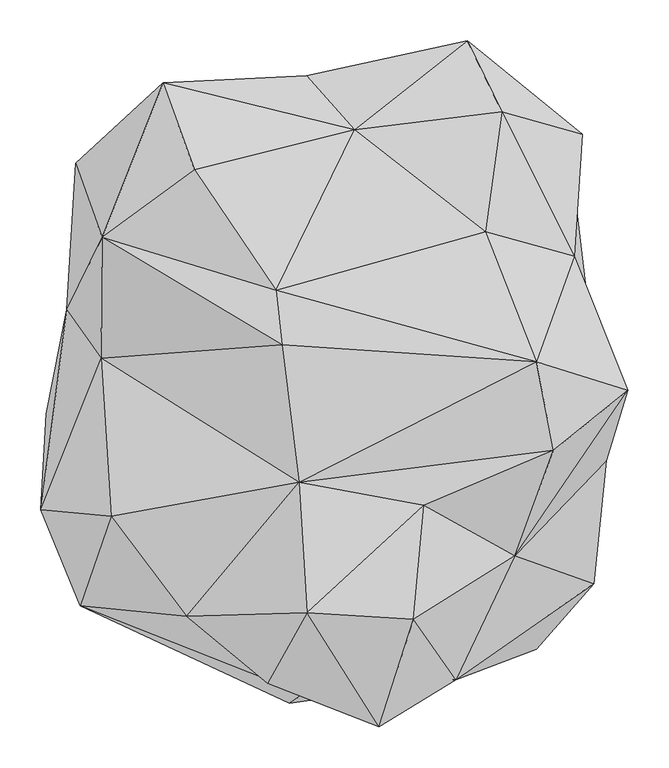
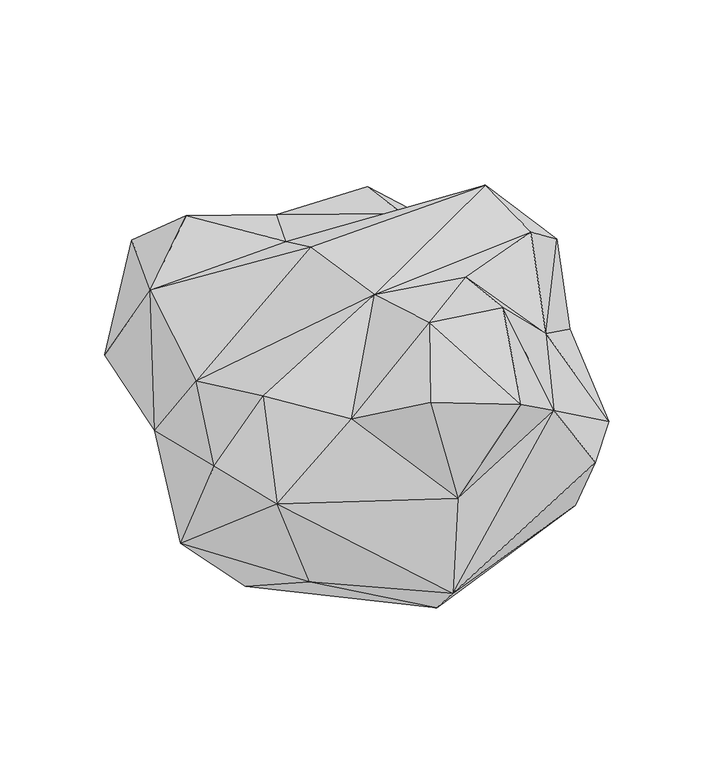
"""IFC4 building model written with IfcOpenShell, lengths in millimetres: geographic element geometry, Enscape AssetDefinition - Asparagaceae 001 Agave : Enscape AssetDefinition - Asparagaceae 001 Agave."""

import ifcopenshell
import ifcopenshell.guid

model = None  # the IFC model being written
_history = None  # IfcOwnerHistory: only IFC2X3 demands one
_inside = {}  # id of a spatial element -> (the spatial element, [elements in it])
_under = {}  # id of a project, library or spatial element -> (it, [spatial elements below it])
_declared = {}  # id of a project -> (the project, [libraries it declares])
_typed = {}  # id of a type object -> (the type object, [elements of that type])
_made_of = {}  # id of a material, layer set ... -> (it, [elements and type objects made of it])


def new_model(schema):
    """Start an empty IFC model of exactly this schema.

    Asked for "IFC4X3", IfcOpenShell would pick the latest addendum, in which some entities
    have other attributes; the version numbers below select the first issue.
    IFC2X3 requires an IfcOwnerHistory on every rooted entity: one is made here for all.
    """
    global model, _history
    if schema == "IFC4X3":
        model = ifcopenshell.file(schema_version=(4, 3, 0, 0))
    else:
        model = ifcopenshell.file(schema=schema)
    _inside.clear()
    _under.clear()
    _declared.clear()
    _typed.clear()
    _made_of.clear()
    _history = None
    if model.schema == "IFC2X3":
        org = make("IfcOrganization", Name="unknown")
        user = make(
            "IfcPersonAndOrganization",
            ThePerson=make("IfcPerson", FamilyName="unknown"),
            TheOrganization=org,
        )
        app = make(
            "IfcApplication",
            ApplicationDeveloper=org,
            Version="unknown",
            ApplicationFullName="unknown",
            ApplicationIdentifier="unknown",
        )
        _history = make(
            "IfcOwnerHistory",
            OwningUser=user,
            OwningApplication=app,
            ChangeAction="ADDED",
            CreationDate=0,
        )
    return model


def make(cls, **values):
    """One entity of the class cls with the attributes given. An attribute that is None is left unset."""
    return model.create_entity(
        cls, **{name: value for name, value in values.items() if value is not None}
    )


def rooted(cls, **values):
    """An entity with a GlobalId (a new one), such as an element, a storey or a relation."""
    return make(cls, GlobalId=ifcopenshell.guid.new(), OwnerHistory=_history, **values)


def si_unit(unit_type, name, prefix=None):
    """IfcSIUnit, for example si_unit("LENGTHUNIT", "METRE", prefix="MILLI")."""
    return make("IfcSIUnit", UnitType=unit_type, Prefix=prefix, Name=name)


def assignment(units):
    """IfcUnitAssignment: the units of a project."""
    return None if units is None else make("IfcUnitAssignment", Units=units)


def point(xyz):
    """IfcCartesianPoint."""
    return None if xyz is None else make("IfcCartesianPoint", Coordinates=xyz)


def direction(xyz):
    """IfcDirection."""
    return None if xyz is None else make("IfcDirection", DirectionRatios=xyz)


def frame(location, z_axis=None, x_axis=None):
    """IfcAxis2Placement3D, a coordinate frame: its origin and axes. An axis left out is left unset."""
    return make(
        "IfcAxis2Placement3D",
        Location=point(location),
        Axis=direction(z_axis),
        RefDirection=direction(x_axis),
    )


def origin():
    """The frame at (0, 0, 0) with its axes left unset."""
    return frame((0.0, 0.0, 0.0))


def place(relative_to, where):
    """IfcLocalPlacement: puts the frame where relative to a parent placement (None: the world)."""
    return make(
        "IfcLocalPlacement", PlacementRelTo=relative_to, RelativePlacement=where
    )


def context(
    kind, dimensions, precision=None, world=None, true_north=None, identifier=None
):
    """IfcGeometricRepresentationContext, for example the 3D "Model" context."""
    return make(
        "IfcGeometricRepresentationContext",
        ContextIdentifier=identifier,
        ContextType=kind,
        CoordinateSpaceDimension=dimensions,
        Precision=precision,
        WorldCoordinateSystem=world,
        TrueNorth=true_north,
    )


def project(units=None, contexts=None):
    """IfcProject with its units and contexts."""
    return rooted(
        "IfcProject",
        Name="project",
        RepresentationContexts=contexts,
        UnitsInContext=assignment(units),
    )


def spatial(cls, under=None, at=None, **own):
    """A site, building, storey or space (cls), placed at a placement, below another one or the project."""
    s = rooted(cls, ObjectPlacement=at, **own)
    if under is not None:
        _under.setdefault(under.id(), (under, []))[1].append(s)
    return s


def faces_of(points, faces, orient=None, outer=None):
    """IfcFace entities. A face is a list of loops; a loop is a list of indices into points, from 0.

    orient and outer hold one flag for each loop. By default every Orientation is true, the
    first loop of a face is its IfcFaceOuterBound and the others are IfcFaceBound.
    """
    made = []
    for i, loops in enumerate(faces):
        bounds = []
        for j, loop in enumerate(loops):
            is_outer = j == 0 if outer is None else outer[i][j]
            bounds.append(
                make(
                    "IfcFaceOuterBound" if is_outer else "IfcFaceBound",
                    Bound=make("IfcPolyLoop", Polygon=[points[k] for k in loop]),
                    Orientation=True if orient is None else orient[i][j],
                )
            )
        made.append(make("IfcFace", Bounds=bounds))
    return made


def faceted_brep(points, faces, orient=None, outer=None, voids=None):
    """IfcFacetedBrep: a solid bounded by flat faces; with voids (closed shells), ...WithVoids."""
    shared = [point(p) for p in points]
    hull = make("IfcClosedShell", CfsFaces=faces_of(shared, faces, orient, outer))
    if voids is None:
        return make("IfcFacetedBrep", Outer=hull)
    return make(
        "IfcFacetedBrepWithVoids",
        Outer=hull,
        Voids=[
            make(cls, CfsFaces=faces_of(shared, fs, o, b)) for cls, fs, o, b in voids
        ],
    )


def shape(context_of_items, identifier, shape_type, items):
    """IfcShapeRepresentation: the items that make up one representation, for example the "Body"."""
    return make(
        "IfcShapeRepresentation",
        ContextOfItems=context_of_items,
        RepresentationIdentifier=identifier,
        RepresentationType=shape_type,
        Items=items,
    )


def source(mapping_origin, context_of_items, identifier, shape_type, items):
    """IfcRepresentationMap: a shape defined once, which mapped items show again and again."""
    return make(
        "IfcRepresentationMap",
        MappingOrigin=mapping_origin,
        MappedRepresentation=shape(context_of_items, identifier, shape_type, items),
    )


def transform(
    local_origin,
    x_axis=None,
    y_axis=None,
    z_axis=None,
    scale=None,
    scale2=None,
    scale3=None,
    uniform=True,
):
    """IfcCartesianTransformationOperator3D, or its non-uniform kind. x_axis, y_axis, z_axis: its Axis1, 2, 3."""
    if uniform:
        return make(
            "IfcCartesianTransformationOperator3D",
            Axis1=direction(x_axis),
            Axis2=direction(y_axis),
            LocalOrigin=point(local_origin),
            Scale=scale,
            Axis3=direction(z_axis),
        )
    return make(
        "IfcCartesianTransformationOperator3DnonUniform",
        Axis1=direction(x_axis),
        Axis2=direction(y_axis),
        LocalOrigin=point(local_origin),
        Scale=scale,
        Axis3=direction(z_axis),
        Scale2=scale2,
        Scale3=scale3,
    )


def mapped(mapping_source, mapping_target):
    """IfcMappedItem: shows the shape of a source again, moved by a transform."""
    return make(
        "IfcMappedItem", MappingSource=mapping_source, MappingTarget=mapping_target
    )


def made_of(thing, what):
    """Note that an element or type object is made of a material, layer set ...; save() writes the relation."""
    if what is not None:
        _made_of.setdefault(what.id(), (what, []))[1].append(thing)
    return thing


def element(
    cls,
    number,
    at=None,
    inside=None,
    cuts=None,
    type_object=None,
    material=None,
    context=None,
    identifier="Body",
    shape_type=None,
    held_by="IfcProductDefinitionShape",
    body=None,
    shapes=None,
    **own,
):
    """One element of the class cls, such as IfcWall. Its Tag is "e" and its number.

    at: its placement. inside: the storey or other place that contains it. cuts: it is an
    opening in that element (IfcRelVoidsElement). A single representation is given by context,
    identifier, shape_type and body (its items); several are given by shapes. held_by: the class
    of the entity that holds the representations. save() writes the other relations.
    """
    e = rooted(cls, Tag="e%d" % number, ObjectPlacement=at, **own)
    if body is not None:
        shapes = [shape(context, identifier, shape_type, body)]
    if shapes is not None:
        e.Representation = make(held_by, Representations=shapes)
    if inside is not None:
        _inside.setdefault(inside.id(), (inside, []))[1].append(e)
    if cuts is not None:
        rooted(
            "IfcRelVoidsElement", RelatingBuildingElement=cuts, RelatedOpeningElement=e
        )
    if type_object is not None:
        _typed.setdefault(type_object.id(), (type_object, []))[1].append(e)
    return made_of(e, material)


def aggregate(whole, parts):
    """IfcRelAggregates: a whole, such as a stair, and the parts it consists of."""
    return rooted("IfcRelAggregates", RelatingObject=whole, RelatedObjects=parts)


def save(model, path):
    """Write the relations noted so far, then the file.

    IfcRelAggregates (storeys below a building ...), IfcRelContainedInSpatialStructure (elements
    in a storey), IfcRelDefinesByType, IfcRelAssociatesMaterial and IfcRelDeclares: one each for
    every whole, place, type object, material and project.
    """
    for whole, parts in _under.values():
        aggregate(whole, parts)
    for where, things in _inside.values():
        rooted(
            "IfcRelContainedInSpatialStructure",
            RelatedElements=things,
            RelatingStructure=where,
        )
    for kind, things in _typed.values():
        rooted("IfcRelDefinesByType", RelatedObjects=things, RelatingType=kind)
    for what, things in _made_of.values():
        rooted("IfcRelAssociatesMaterial", RelatedObjects=things, RelatingMaterial=what)
    for by, libraries in _declared.values():
        rooted("IfcRelDeclares", RelatingContext=by, RelatedDefinitions=libraries)
    model.write(path)


def geographic_element_a6fbcd7a(model_context):
    return source(origin(), model_context, "Body", "Brep", [
        faceted_brep([(-83.9166865, 203.263849, 0.0), (12.647056, 313.811481, 48.0152518), (67.6679313, 62.6604483, 0.0), (180.0118238, 64.2274469, 0.0), (-240.9703434, 321.6060698, 224.4298905), (218.8661695, 340.318799, 147.609368), (130.1935166, 418.3222353, 188.9963597), (54.3873757, -37.3966545, 0.0), (-309.7500205, 30.4520428, 66.9589713), (-282.8032076, -74.3769556, 51.3344258), (-68.5941651, -314.8398399, 80.1332444), (281.7476392, -32.8720361, 60.0785054), (227.4366021, -243.2648838, 132.4731708), (-372.3214567, -22.7501001, 135.3752464), (-245.0786829, -213.5978639, 130.9934407), (-74.6905804, -376.1395216, 147.9662508), (297.0918119, -230.159983, 264.4174993), (226.5083939, -310.1032972, 257.6498091), (-58.5948005, -364.6009266, 320.3084469), (-330.3538561, -257.1682334, 339.8004174), (128.2582879, -347.3773599, 415.8658981), (-292.5794125, -147.57514, 469.5923924), (-378.6310256, -139.8030221, 359.0724468), (-200.5006969, -269.4469392, 466.7710066), (-101.5319452, -351.2604833, 514.261961), (34.3744606, -404.9287438, 495.1784015), (-53.6577664, -265.4434741, 601.4473438), (-63.4572953, -105.9724018, 562.3546839), (-305.0922155, 45.468282, 386.8079782), (-347.0320106, 104.5354754, 268.994689), (-303.935796, 193.1274682, 474.0562737), (-84.1022134, 61.705336, 560.44662), (-336.4052773, 283.3358645, 304.1164875), (-91.2186354, 128.3842325, 533.411622), (-190.626651, 275.4265964, 529.8674107), (-229.4352949, 381.8665445, 430.6333363), (226.3577729, 40.6467356, 585.7200027), (164.413169, 199.5292455, 455.4721117), (4.5721261, 324.2405057, 433.6276054), (-53.8770929, 389.9331093, 315.5574501), (-227.6405096, 376.0583401, 284.8320007), (142.7014321, 432.5819612, 292.3455834), (184.7079694, 346.2255597, 411.3186896), (272.7532089, 169.5409268, 383.0037415), (283.0359936, 318.8481033, 317.0358241), (273.9757001, 240.0513738, 187.9213154), (338.1246328, 6.1014961, 462.3352885), (312.279731, -80.1761523, 348.0335176), (200.6652653, -196.0080713, 448.3486712), (247.2611368, -67.0667812, 551.8904924), (89.1786218, -134.4338804, 560.2785349), (76.2959495, -273.5785842, 589.6103978)], [[[0, 1, 2]], [[2, 1, 3]], [[4, 1, 0]], [[1, 5, 3]], [[1, 6, 5]], [[1, 4, 6]], [[7, 0, 2]], [[7, 2, 3]], [[4, 0, 8]], [[8, 0, 7]], [[9, 7, 10]], [[7, 11, 12]], [[11, 7, 3]], [[9, 8, 7]], [[12, 10, 7]], [[8, 13, 4]], [[13, 8, 9]], [[9, 14, 13]], [[14, 9, 10]], [[10, 12, 15]], [[10, 15, 14]], [[11, 16, 12]], [[12, 17, 15]], [[17, 12, 16]], [[15, 18, 19]], [[14, 15, 19]], [[17, 20, 15]], [[18, 15, 20]], [[13, 14, 19]], [[21, 22, 19]], [[22, 13, 19]], [[18, 23, 19]], [[21, 19, 23]], [[18, 24, 23]], [[18, 25, 24]], [[18, 20, 25]], [[23, 24, 26]], [[23, 26, 27]], [[21, 23, 27]], [[21, 28, 22]], [[21, 27, 28]], [[28, 29, 22]], [[13, 22, 29]], [[28, 30, 29]], [[30, 28, 31]], [[27, 31, 28]], [[4, 29, 32]], [[29, 4, 13]], [[29, 30, 32]], [[30, 33, 34]], [[35, 30, 34]], [[30, 31, 33]], [[32, 30, 35]], [[31, 36, 33]], [[27, 36, 31]], [[37, 38, 33]], [[33, 36, 37]], [[34, 33, 38]], [[34, 38, 35]], [[39, 35, 38]], [[32, 35, 40]], [[40, 35, 39]], [[4, 32, 40]], [[4, 40, 39]], [[4, 39, 6]], [[39, 41, 6]], [[39, 38, 41]], [[38, 42, 41]], [[38, 37, 42]], [[37, 36, 43]], [[43, 42, 37]], [[41, 42, 44]], [[43, 44, 42]], [[6, 41, 5]], [[5, 41, 44]], [[44, 45, 5]], [[45, 44, 43]], [[46, 47, 43]], [[43, 36, 46]], [[47, 45, 43]], [[5, 45, 3]], [[11, 3, 45]], [[11, 45, 47]], [[47, 46, 48]], [[48, 16, 47]], [[16, 11, 47]], [[48, 46, 49]], [[46, 36, 49]], [[27, 49, 36]], [[49, 50, 48]], [[50, 49, 27]], [[48, 51, 20]], [[51, 48, 50]], [[20, 16, 48]], [[20, 17, 16]], [[20, 51, 25]], [[50, 26, 51]], [[26, 25, 51]], [[26, 50, 27]], [[24, 25, 26]]]),
    ])


if __name__ == "__main__":
    model = new_model("IFC4")
    model_context = context("Model", 3, world=origin())
    ifc_project = project(units=[si_unit("LENGTHUNIT", "METRE", prefix="MILLI")], contexts=[model_context])
    site = spatial("IfcSite", under=ifc_project)
    building = spatial("IfcBuilding", under=site)
    placement = place(None, origin())
    geographic_element_shape = geographic_element_a6fbcd7a(model_context)
    element("IfcGeographicElement", 1, ObjectType="Enscape AssetDefinition - Asparagaceae 001 Agave : Enscape AssetDefinition - Asparagaceae 001 Agave", at=placement, inside=building, context=model_context, shape_type="MappedRepresentation", body=[
        mapped(geographic_element_shape, transform((0.0, 0.0, 0.0), x_axis=(1.0, 0.0, 0.0), y_axis=(0.0, 1.0, 0.0), z_axis=(0.0, 0.0, 1.0))),
    ])
    save(model, "model.ifc")

# Revit data of these elements
# Type "Enscape AssetDefinition - Asparagaceae 001 Agave : Enscape AssetDefinition - Asparagaceae 001 Agave"
#   EnscapeAssetSource = "REMOTE"
#   EnscapeAssetId = "6d861ce6-d1f1-4992-8acd-35a045128a82"
#   Height = 0.601447 m
#   EnscapeNativeAssetHeight = 0.601447 m
#   Default Elevation = 0
